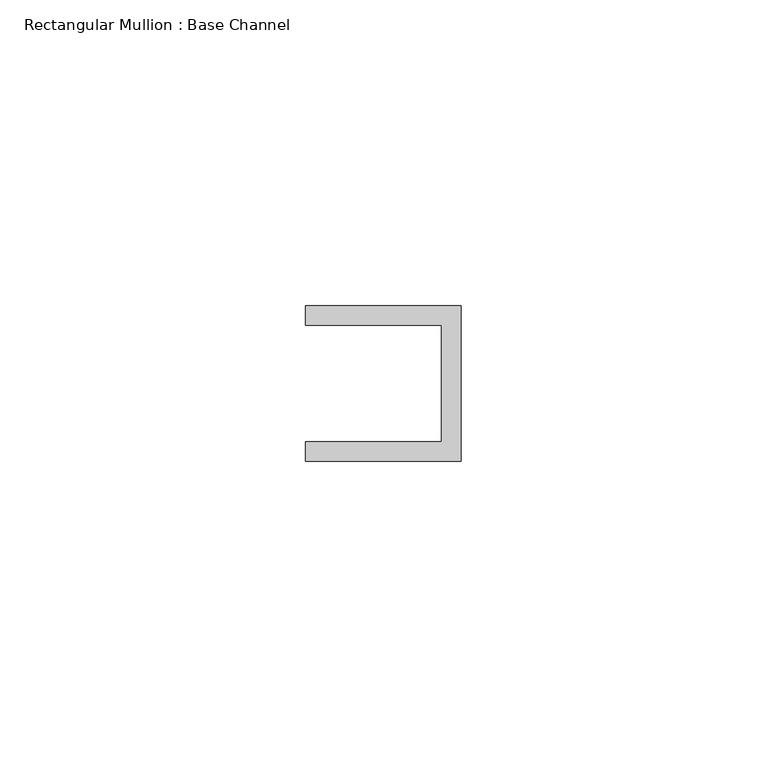
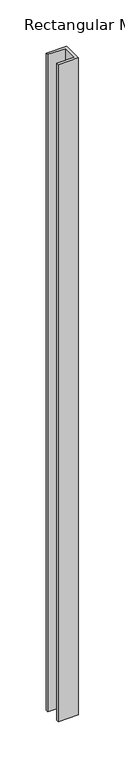
"""IFC4 building model written with IfcOpenShell, lengths in millimetres: member geometry, Rectangular Mullion : Base Channel."""

import ifcopenshell
import ifcopenshell.guid

model = None  # the IFC model being written
_history = None  # IfcOwnerHistory: only IFC2X3 demands one
_inside = {}  # id of a spatial element -> (the spatial element, [elements in it])
_under = {}  # id of a project, library or spatial element -> (it, [spatial elements below it])
_declared = {}  # id of a project -> (the project, [libraries it declares])
_typed = {}  # id of a type object -> (the type object, [elements of that type])
_made_of = {}  # id of a material, layer set ... -> (it, [elements and type objects made of it])


def new_model(schema):
    """Start an empty IFC model of exactly this schema.

    Asked for "IFC4X3", IfcOpenShell would pick the latest addendum, in which some entities
    have other attributes; the version numbers below select the first issue.
    IFC2X3 requires an IfcOwnerHistory on every rooted entity: one is made here for all.
    """
    global model, _history
    if schema == "IFC4X3":
        model = ifcopenshell.file(schema_version=(4, 3, 0, 0))
    else:
        model = ifcopenshell.file(schema=schema)
    _inside.clear()
    _under.clear()
    _declared.clear()
    _typed.clear()
    _made_of.clear()
    _history = None
    if model.schema == "IFC2X3":
        org = make("IfcOrganization", Name="unknown")
        user = make(
            "IfcPersonAndOrganization",
            ThePerson=make("IfcPerson", FamilyName="unknown"),
            TheOrganization=org,
        )
        app = make(
            "IfcApplication",
            ApplicationDeveloper=org,
            Version="unknown",
            ApplicationFullName="unknown",
            ApplicationIdentifier="unknown",
        )
        _history = make(
            "IfcOwnerHistory",
            OwningUser=user,
            OwningApplication=app,
            ChangeAction="ADDED",
            CreationDate=0,
        )
    return model


def make(cls, **values):
    """One entity of the class cls with the attributes given. An attribute that is None is left unset."""
    return model.create_entity(
        cls, **{name: value for name, value in values.items() if value is not None}
    )


def rooted(cls, **values):
    """An entity with a GlobalId (a new one), such as an element, a storey or a relation."""
    return make(cls, GlobalId=ifcopenshell.guid.new(), OwnerHistory=_history, **values)


def si_unit(unit_type, name, prefix=None):
    """IfcSIUnit, for example si_unit("LENGTHUNIT", "METRE", prefix="MILLI")."""
    return make("IfcSIUnit", UnitType=unit_type, Prefix=prefix, Name=name)


def assignment(units):
    """IfcUnitAssignment: the units of a project."""
    return None if units is None else make("IfcUnitAssignment", Units=units)


def point(xyz):
    """IfcCartesianPoint."""
    return None if xyz is None else make("IfcCartesianPoint", Coordinates=xyz)


def direction(xyz):
    """IfcDirection."""
    return None if xyz is None else make("IfcDirection", DirectionRatios=xyz)


def frame(location, z_axis=None, x_axis=None):
    """IfcAxis2Placement3D, a coordinate frame: its origin and axes. An axis left out is left unset."""
    return make(
        "IfcAxis2Placement3D",
        Location=point(location),
        Axis=direction(z_axis),
        RefDirection=direction(x_axis),
    )


def origin():
    """The frame at (0, 0, 0) with its axes left unset."""
    return frame((0.0, 0.0, 0.0))


def place(relative_to, where):
    """IfcLocalPlacement: puts the frame where relative to a parent placement (None: the world)."""
    return make(
        "IfcLocalPlacement", PlacementRelTo=relative_to, RelativePlacement=where
    )


def context(
    kind, dimensions, precision=None, world=None, true_north=None, identifier=None
):
    """IfcGeometricRepresentationContext, for example the 3D "Model" context."""
    return make(
        "IfcGeometricRepresentationContext",
        ContextIdentifier=identifier,
        ContextType=kind,
        CoordinateSpaceDimension=dimensions,
        Precision=precision,
        WorldCoordinateSystem=world,
        TrueNorth=true_north,
    )


def project(units=None, contexts=None):
    """IfcProject with its units and contexts."""
    return rooted(
        "IfcProject",
        Name="project",
        RepresentationContexts=contexts,
        UnitsInContext=assignment(units),
    )


def spatial(cls, under=None, at=None, **own):
    """A site, building, storey or space (cls), placed at a placement, below another one or the project."""
    s = rooted(cls, ObjectPlacement=at, **own)
    if under is not None:
        _under.setdefault(under.id(), (under, []))[1].append(s)
    return s


def polyline(points):
    """IfcPolyline through the points."""
    return make("IfcPolyline", Points=[point(p) for p in points])


def outline(outer, holes=None, kind="AREA"):
    """IfcArbitraryClosedProfileDef: a profile drawn as a closed curve; with holes, ...WithVoids."""
    if holes is None:
        return make("IfcArbitraryClosedProfileDef", ProfileType=kind, OuterCurve=outer)
    return make(
        "IfcArbitraryProfileDefWithVoids",
        ProfileType=kind,
        OuterCurve=outer,
        InnerCurves=holes,
    )


def extrude(swept, where, along, depth):
    """IfcExtrudedAreaSolid: the profile swept, set in the frame where, extruded along a direction by depth."""
    return make(
        "IfcExtrudedAreaSolid",
        SweptArea=swept,
        Position=where,
        ExtrudedDirection=direction(along),
        Depth=depth,
    )


def shape(context_of_items, identifier, shape_type, items):
    """IfcShapeRepresentation: the items that make up one representation, for example the "Body"."""
    return make(
        "IfcShapeRepresentation",
        ContextOfItems=context_of_items,
        RepresentationIdentifier=identifier,
        RepresentationType=shape_type,
        Items=items,
    )


def source(mapping_origin, context_of_items, identifier, shape_type, items):
    """IfcRepresentationMap: a shape defined once, which mapped items show again and again."""
    return make(
        "IfcRepresentationMap",
        MappingOrigin=mapping_origin,
        MappedRepresentation=shape(context_of_items, identifier, shape_type, items),
    )


def transform(
    local_origin,
    x_axis=None,
    y_axis=None,
    z_axis=None,
    scale=None,
    scale2=None,
    scale3=None,
    uniform=True,
):
    """IfcCartesianTransformationOperator3D, or its non-uniform kind. x_axis, y_axis, z_axis: its Axis1, 2, 3."""
    if uniform:
        return make(
            "IfcCartesianTransformationOperator3D",
            Axis1=direction(x_axis),
            Axis2=direction(y_axis),
            LocalOrigin=point(local_origin),
            Scale=scale,
            Axis3=direction(z_axis),
        )
    return make(
        "IfcCartesianTransformationOperator3DnonUniform",
        Axis1=direction(x_axis),
        Axis2=direction(y_axis),
        LocalOrigin=point(local_origin),
        Scale=scale,
        Axis3=direction(z_axis),
        Scale2=scale2,
        Scale3=scale3,
    )


def mapped(mapping_source, mapping_target):
    """IfcMappedItem: shows the shape of a source again, moved by a transform."""
    return make(
        "IfcMappedItem", MappingSource=mapping_source, MappingTarget=mapping_target
    )


def made_of(thing, what):
    """Note that an element or type object is made of a material, layer set ...; save() writes the relation."""
    if what is not None:
        _made_of.setdefault(what.id(), (what, []))[1].append(thing)
    return thing


def element(
    cls,
    number,
    at=None,
    inside=None,
    cuts=None,
    type_object=None,
    material=None,
    context=None,
    identifier="Body",
    shape_type=None,
    held_by="IfcProductDefinitionShape",
    body=None,
    shapes=None,
    **own,
):
    """One element of the class cls, such as IfcWall. Its Tag is "e" and its number.

    at: its placement. inside: the storey or other place that contains it. cuts: it is an
    opening in that element (IfcRelVoidsElement). A single representation is given by context,
    identifier, shape_type and body (its items); several are given by shapes. held_by: the class
    of the entity that holds the representations. save() writes the other relations.
    """
    e = rooted(cls, Tag="e%d" % number, ObjectPlacement=at, **own)
    if body is not None:
        shapes = [shape(context, identifier, shape_type, body)]
    if shapes is not None:
        e.Representation = make(held_by, Representations=shapes)
    if inside is not None:
        _inside.setdefault(inside.id(), (inside, []))[1].append(e)
    if cuts is not None:
        rooted(
            "IfcRelVoidsElement", RelatingBuildingElement=cuts, RelatedOpeningElement=e
        )
    if type_object is not None:
        _typed.setdefault(type_object.id(), (type_object, []))[1].append(e)
    return made_of(e, material)


def aggregate(whole, parts):
    """IfcRelAggregates: a whole, such as a stair, and the parts it consists of."""
    return rooted("IfcRelAggregates", RelatingObject=whole, RelatedObjects=parts)


def save(model, path):
    """Write the relations noted so far, then the file.

    IfcRelAggregates (storeys below a building ...), IfcRelContainedInSpatialStructure (elements
    in a storey), IfcRelDefinesByType, IfcRelAssociatesMaterial and IfcRelDeclares: one each for
    every whole, place, type object, material and project.
    """
    for whole, parts in _under.values():
        aggregate(whole, parts)
    for where, things in _inside.values():
        rooted(
            "IfcRelContainedInSpatialStructure",
            RelatedElements=things,
            RelatingStructure=where,
        )
    for kind, things in _typed.values():
        rooted("IfcRelDefinesByType", RelatedObjects=things, RelatingType=kind)
    for what, things in _made_of.values():
        rooted("IfcRelAssociatesMaterial", RelatedObjects=things, RelatingMaterial=what)
    for by, libraries in _declared.values():
        rooted("IfcRelDeclares", RelatingContext=by, RelatedDefinitions=libraries)
    model.write(path)


def rectangular_mullion_base_channel_eb5970c3(model_context):
    return source(origin(), model_context, "Body", "SweptSolid", [
        extrude(outline(polyline([(0.0, 12.7), (0.0, -12.7), (-25.4, -12.7), (-25.4, -9.525), (-3.175, -9.525), (-3.175, 9.525), (-25.4, 9.525), (-25.4, 12.7), (0.0, 12.7)])), frame((0.0, 0.0, -866.775), z_axis=(0.0, 0.0, 1.0), x_axis=(1.0, 0.0, 0.0)), (0.0, 0.0, 1.0), 866.775),
    ])


if __name__ == "__main__":
    model = new_model("IFC4")
    model_context = context("Model", 3, world=origin())
    ifc_project = project(units=[si_unit("LENGTHUNIT", "METRE", prefix="MILLI")], contexts=[model_context])
    site = spatial("IfcSite", under=ifc_project)
    building = spatial("IfcBuilding", under=site)
    placement = place(None, origin())
    rectangular_mullion_base_channel_shape = rectangular_mullion_base_channel_eb5970c3(model_context)
    element("IfcMember", 1, ObjectType="Rectangular Mullion : Base Channel", at=placement, inside=building, context=model_context, shape_type="MappedRepresentation", body=[
        mapped(rectangular_mullion_base_channel_shape, transform((0.0, 0.0, 0.0), x_axis=(1.0, 0.0, 0.0), y_axis=(0.0, 1.0, 0.0), z_axis=(0.0, 0.0, 1.0))),
    ])
    save(model, "model.ifc")

# Revit data of these elements
# Type "Rectangular Mullion : Base Channel"
#   built-in parameter 1007322 = 0.0833333 (stored number, unit not read)
#   built-in parameter 1007321 = 0.0416667 (stored number, unit not read)
#   built-in parameter 1007320 = -0.03125 (stored number, unit not read)
# Element 1 (IfcMember, "Rectangular Mullion : Base Channel")
#   Materials on its faces: "ALUM"
# Materials
#   "ALUM": class "Generic", colour RGB 157 157 157, transparency 0, Cost = 0
